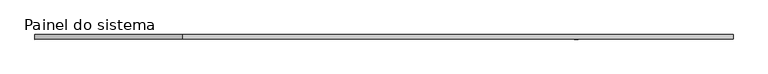
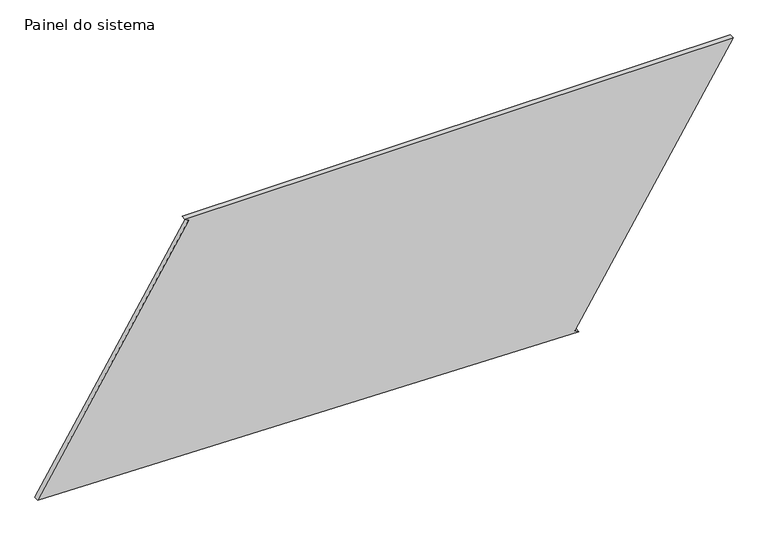
"""IFC4 building model written with IfcOpenShell, lengths in millimetres: plate geometry, Painel do sistema : Envidraçado."""

from ifc_helpers import new_model, si_unit, frame, origin, place, context, project, spatial, polyline, outline, extrude, source, transform, mapped, element, save


def painel_do_sistema_c6a056eb(model_context):
    return source(origin(), model_context, "Body", "SweptSolid", [
        extrude(outline(polyline([(0.0, 1058.3279508), (13.2016257, 1037.0978524), (1405.405402, 1902.8193767), (1405.405402, -1097.2007931), (1392.2037763, -1075.9706947), (62.5130787, -1902.8193767), (0.0, 1058.3279508)])), frame((0.0, 24.5, 0.0), z_axis=(0.0, 1.0, 0.0), x_axis=(0.0, 0.0, 1.0)), (0.0, 0.0, 1.0), 25.0),
    ])


if __name__ == "__main__":
    model = new_model("IFC4")
    model_context = context("Model", 3, world=origin())
    ifc_project = project(units=[si_unit("LENGTHUNIT", "METRE", prefix="MILLI")], contexts=[model_context])
    site = spatial("IfcSite", under=ifc_project)
    building = spatial("IfcBuilding", under=site)
    placement = place(None, origin())
    painel_do_sistema_shape = painel_do_sistema_c6a056eb(model_context)
    element("IfcPlate", 1, ObjectType="Painel do sistema : Envidraçado", at=placement, inside=building, context=model_context, shape_type="MappedRepresentation", body=[
        mapped(painel_do_sistema_shape, transform((0.0, 0.0, 0.0), x_axis=(1.0, 0.0, 0.0), y_axis=(0.0, 1.0, 0.0), z_axis=(0.0, 0.0, 1.0))),
    ])
    save(model, "model.ifc")

# Revit data of these elements
# Type "Painel do sistema : Envidraçado"
#   Construction Type Id = "GSP4R"
#   Analytic Construction = "Vidraça única Pilkington 1/8 pol"
#   Visual Light Transmittance = 0.9
#   Solar Heat Gain Coefficient = 0.86
#   Heat Transfer Coefficient (U) = 6.7069 W/(m²·K)
# Element 1 (IfcPlate, "Painel do sistema : Envidraçado")
#   Materials on its faces: "Vidro"
# Materials
#   "Vidro": class "Vidro", colour RGB 0 128 192, transparency 0.9, Description = "Vidro de sílica", Cost = 0
